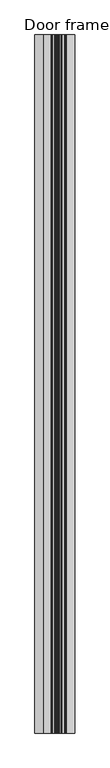
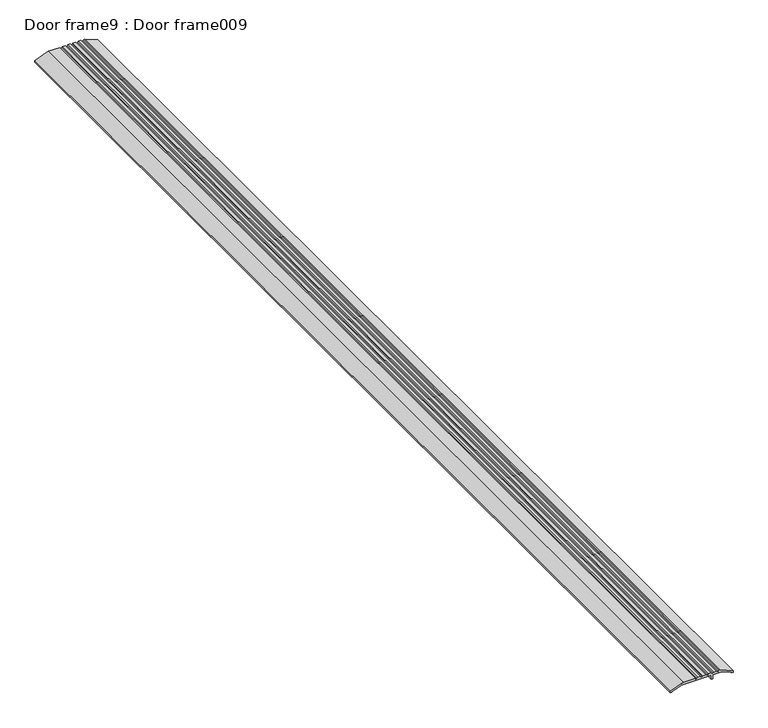
"""IFC4 building model written with IfcOpenShell, lengths in millimetres: proxy geometry, Door frame9 : Door frame009."""

import ifcopenshell
import ifcopenshell.guid

model = None  # the IFC model being written
_history = None  # IfcOwnerHistory: only IFC2X3 demands one
_inside = {}  # id of a spatial element -> (the spatial element, [elements in it])
_under = {}  # id of a project, library or spatial element -> (it, [spatial elements below it])
_declared = {}  # id of a project -> (the project, [libraries it declares])
_typed = {}  # id of a type object -> (the type object, [elements of that type])
_made_of = {}  # id of a material, layer set ... -> (it, [elements and type objects made of it])


def new_model(schema):
    """Start an empty IFC model of exactly this schema.

    Asked for "IFC4X3", IfcOpenShell would pick the latest addendum, in which some entities
    have other attributes; the version numbers below select the first issue.
    IFC2X3 requires an IfcOwnerHistory on every rooted entity: one is made here for all.
    """
    global model, _history
    if schema == "IFC4X3":
        model = ifcopenshell.file(schema_version=(4, 3, 0, 0))
    else:
        model = ifcopenshell.file(schema=schema)
    _inside.clear()
    _under.clear()
    _declared.clear()
    _typed.clear()
    _made_of.clear()
    _history = None
    if model.schema == "IFC2X3":
        org = make("IfcOrganization", Name="unknown")
        user = make(
            "IfcPersonAndOrganization",
            ThePerson=make("IfcPerson", FamilyName="unknown"),
            TheOrganization=org,
        )
        app = make(
            "IfcApplication",
            ApplicationDeveloper=org,
            Version="unknown",
            ApplicationFullName="unknown",
            ApplicationIdentifier="unknown",
        )
        _history = make(
            "IfcOwnerHistory",
            OwningUser=user,
            OwningApplication=app,
            ChangeAction="ADDED",
            CreationDate=0,
        )
    return model


def make(cls, **values):
    """One entity of the class cls with the attributes given. An attribute that is None is left unset."""
    return model.create_entity(
        cls, **{name: value for name, value in values.items() if value is not None}
    )


def rooted(cls, **values):
    """An entity with a GlobalId (a new one), such as an element, a storey or a relation."""
    return make(cls, GlobalId=ifcopenshell.guid.new(), OwnerHistory=_history, **values)


def si_unit(unit_type, name, prefix=None):
    """IfcSIUnit, for example si_unit("LENGTHUNIT", "METRE", prefix="MILLI")."""
    return make("IfcSIUnit", UnitType=unit_type, Prefix=prefix, Name=name)


def assignment(units):
    """IfcUnitAssignment: the units of a project."""
    return None if units is None else make("IfcUnitAssignment", Units=units)


def point(xyz):
    """IfcCartesianPoint."""
    return None if xyz is None else make("IfcCartesianPoint", Coordinates=xyz)


def direction(xyz):
    """IfcDirection."""
    return None if xyz is None else make("IfcDirection", DirectionRatios=xyz)


def frame(location, z_axis=None, x_axis=None):
    """IfcAxis2Placement3D, a coordinate frame: its origin and axes. An axis left out is left unset."""
    return make(
        "IfcAxis2Placement3D",
        Location=point(location),
        Axis=direction(z_axis),
        RefDirection=direction(x_axis),
    )


def origin():
    """The frame at (0, 0, 0) with its axes left unset."""
    return frame((0.0, 0.0, 0.0))


def place(relative_to, where):
    """IfcLocalPlacement: puts the frame where relative to a parent placement (None: the world)."""
    return make(
        "IfcLocalPlacement", PlacementRelTo=relative_to, RelativePlacement=where
    )


def context(
    kind, dimensions, precision=None, world=None, true_north=None, identifier=None
):
    """IfcGeometricRepresentationContext, for example the 3D "Model" context."""
    return make(
        "IfcGeometricRepresentationContext",
        ContextIdentifier=identifier,
        ContextType=kind,
        CoordinateSpaceDimension=dimensions,
        Precision=precision,
        WorldCoordinateSystem=world,
        TrueNorth=true_north,
    )


def project(units=None, contexts=None):
    """IfcProject with its units and contexts."""
    return rooted(
        "IfcProject",
        Name="project",
        RepresentationContexts=contexts,
        UnitsInContext=assignment(units),
    )


def spatial(cls, under=None, at=None, **own):
    """A site, building, storey or space (cls), placed at a placement, below another one or the project."""
    s = rooted(cls, ObjectPlacement=at, **own)
    if under is not None:
        _under.setdefault(under.id(), (under, []))[1].append(s)
    return s


def polyline(points):
    """IfcPolyline through the points."""
    return make("IfcPolyline", Points=[point(p) for p in points])


def outline(outer, holes=None, kind="AREA"):
    """IfcArbitraryClosedProfileDef: a profile drawn as a closed curve; with holes, ...WithVoids."""
    if holes is None:
        return make("IfcArbitraryClosedProfileDef", ProfileType=kind, OuterCurve=outer)
    return make(
        "IfcArbitraryProfileDefWithVoids",
        ProfileType=kind,
        OuterCurve=outer,
        InnerCurves=holes,
    )


def extrude(swept, where, along, depth):
    """IfcExtrudedAreaSolid: the profile swept, set in the frame where, extruded along a direction by depth."""
    return make(
        "IfcExtrudedAreaSolid",
        SweptArea=swept,
        Position=where,
        ExtrudedDirection=direction(along),
        Depth=depth,
    )


def shape(context_of_items, identifier, shape_type, items):
    """IfcShapeRepresentation: the items that make up one representation, for example the "Body"."""
    return make(
        "IfcShapeRepresentation",
        ContextOfItems=context_of_items,
        RepresentationIdentifier=identifier,
        RepresentationType=shape_type,
        Items=items,
    )


def source(mapping_origin, context_of_items, identifier, shape_type, items):
    """IfcRepresentationMap: a shape defined once, which mapped items show again and again."""
    return make(
        "IfcRepresentationMap",
        MappingOrigin=mapping_origin,
        MappedRepresentation=shape(context_of_items, identifier, shape_type, items),
    )


def transform(
    local_origin,
    x_axis=None,
    y_axis=None,
    z_axis=None,
    scale=None,
    scale2=None,
    scale3=None,
    uniform=True,
):
    """IfcCartesianTransformationOperator3D, or its non-uniform kind. x_axis, y_axis, z_axis: its Axis1, 2, 3."""
    if uniform:
        return make(
            "IfcCartesianTransformationOperator3D",
            Axis1=direction(x_axis),
            Axis2=direction(y_axis),
            LocalOrigin=point(local_origin),
            Scale=scale,
            Axis3=direction(z_axis),
        )
    return make(
        "IfcCartesianTransformationOperator3DnonUniform",
        Axis1=direction(x_axis),
        Axis2=direction(y_axis),
        LocalOrigin=point(local_origin),
        Scale=scale,
        Axis3=direction(z_axis),
        Scale2=scale2,
        Scale3=scale3,
    )


def mapped(mapping_source, mapping_target):
    """IfcMappedItem: shows the shape of a source again, moved by a transform."""
    return make(
        "IfcMappedItem", MappingSource=mapping_source, MappingTarget=mapping_target
    )


def made_of(thing, what):
    """Note that an element or type object is made of a material, layer set ...; save() writes the relation."""
    if what is not None:
        _made_of.setdefault(what.id(), (what, []))[1].append(thing)
    return thing


def element(
    cls,
    number,
    at=None,
    inside=None,
    cuts=None,
    type_object=None,
    material=None,
    context=None,
    identifier="Body",
    shape_type=None,
    held_by="IfcProductDefinitionShape",
    body=None,
    shapes=None,
    **own,
):
    """One element of the class cls, such as IfcWall. Its Tag is "e" and its number.

    at: its placement. inside: the storey or other place that contains it. cuts: it is an
    opening in that element (IfcRelVoidsElement). A single representation is given by context,
    identifier, shape_type and body (its items); several are given by shapes. held_by: the class
    of the entity that holds the representations. save() writes the other relations.
    """
    e = rooted(cls, Tag="e%d" % number, ObjectPlacement=at, **own)
    if body is not None:
        shapes = [shape(context, identifier, shape_type, body)]
    if shapes is not None:
        e.Representation = make(held_by, Representations=shapes)
    if inside is not None:
        _inside.setdefault(inside.id(), (inside, []))[1].append(e)
    if cuts is not None:
        rooted(
            "IfcRelVoidsElement", RelatingBuildingElement=cuts, RelatedOpeningElement=e
        )
    if type_object is not None:
        _typed.setdefault(type_object.id(), (type_object, []))[1].append(e)
    return made_of(e, material)


def aggregate(whole, parts):
    """IfcRelAggregates: a whole, such as a stair, and the parts it consists of."""
    return rooted("IfcRelAggregates", RelatingObject=whole, RelatedObjects=parts)


def save(model, path):
    """Write the relations noted so far, then the file.

    IfcRelAggregates (storeys below a building ...), IfcRelContainedInSpatialStructure (elements
    in a storey), IfcRelDefinesByType, IfcRelAssociatesMaterial and IfcRelDeclares: one each for
    every whole, place, type object, material and project.
    """
    for whole, parts in _under.values():
        aggregate(whole, parts)
    for where, things in _inside.values():
        rooted(
            "IfcRelContainedInSpatialStructure",
            RelatedElements=things,
            RelatingStructure=where,
        )
    for kind, things in _typed.values():
        rooted("IfcRelDefinesByType", RelatedObjects=things, RelatingType=kind)
    for what, things in _made_of.values():
        rooted("IfcRelAssociatesMaterial", RelatedObjects=things, RelatingMaterial=what)
    for by, libraries in _declared.values():
        rooted("IfcRelDeclares", RelatingContext=by, RelatedDefinitions=libraries)
    model.write(path)


def door_frame9_door_frame009_747449c1(model_context):
    return source(origin(), model_context, "Body", "SweptSolid", [
        extrude(outline(polyline([(36582.0975353, 15569.2471527), (36582.0975353, 15564.3576527), (36580.0353123, 15563.1670277), (36580.0353123, 15560.7857777), (36582.0975353, 15559.5951527), (36582.0975353, 15554.7056527), (36580.0353123, 15553.5150277), (36580.0353123, 15551.1337777), (36582.0975353, 15549.9431527), (36582.0975353, 15528.6904507), (36572.5243303, 15504.8264027), (36569.3983841, 15504.8264027), (36569.3983841, 15508.0014027), (36570.3770561, 15508.0014027), (36577.3350353, 15525.3462262), (36577.3350353, 15579.7549595), (36569.5937593, 15579.7549595), (36569.5937593, 15582.2978458), (36577.3350353, 15582.2978458), (36577.3350353, 15598.6065792), (36570.3770561, 15615.9514027), (36569.3983841, 15615.9514027), (36569.3983841, 15619.1264027), (36572.5243303, 15619.1264027), (36582.0975353, 15595.2623546), (36582.0975353, 15593.3136527), (36580.0353123, 15592.1230277), (36580.0353123, 15589.7417777), (36582.0975353, 15588.5511527), (36582.0975353, 15583.6616527), (36580.0353123, 15582.4710277), (36580.0353123, 15580.0897777), (36582.0975353, 15578.8991527), (36582.0975353, 15574.0096527), (36580.0353123, 15572.8190277), (36580.0353123, 15570.4377777), (36582.0975353, 15569.2471527)])), frame((0.0, -1052.8906567, 0.0), z_axis=(0.0, 1.0, 0.0), x_axis=(0.0, 0.0, 1.0)), (0.0, 0.0, 1.0), 1999.85),
    ])


if __name__ == "__main__":
    model = new_model("IFC4")
    model_context = context("Model", 3, world=origin())
    ifc_project = project(units=[si_unit("LENGTHUNIT", "METRE", prefix="MILLI")], contexts=[model_context])
    site = spatial("IfcSite", under=ifc_project)
    building = spatial("IfcBuilding", under=site)
    placement = place(None, origin())
    door_frame9_door_frame009_shape = door_frame9_door_frame009_747449c1(model_context)
    element("IfcBuildingElementProxy", 1, Name="Door frame9 : Door frame009", ObjectType="Door frame9 : Door frame009", at=placement, inside=building, context=model_context, shape_type="MappedRepresentation", body=[
        mapped(door_frame9_door_frame009_shape, transform((0.0, 0.0, 0.0), x_axis=(1.0, 0.0, 0.0), y_axis=(0.0, 1.0, 0.0), z_axis=(0.0, 0.0, 1.0))),
    ])
    save(model, "model.ifc")

# Revit data of these elements
# Type "Door frame9 : Door frame009"
#   NameOverride = "Door frame009"
# Element 1 (IfcBuildingElementProxy, "Door frame9 : Door frame009")
#   Materials on its faces: "ALUM. THRESHOLD"
# Materials
#   "ALUM. THRESHOLD": class "Metal", colour RGB 247 247 247, transparency 0, Description = "Aluminum 6061", Cost = 0
